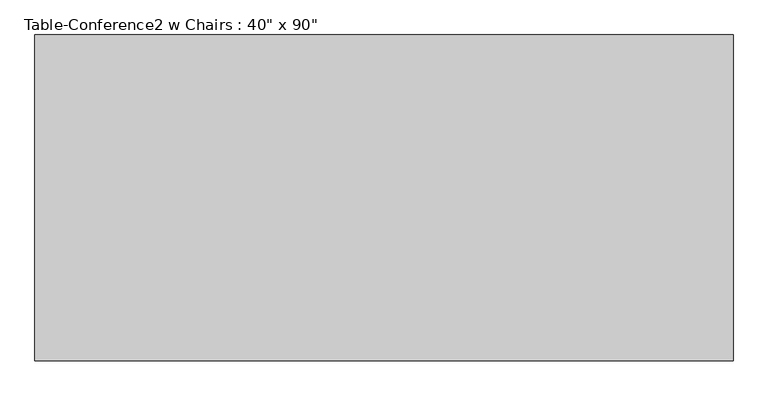
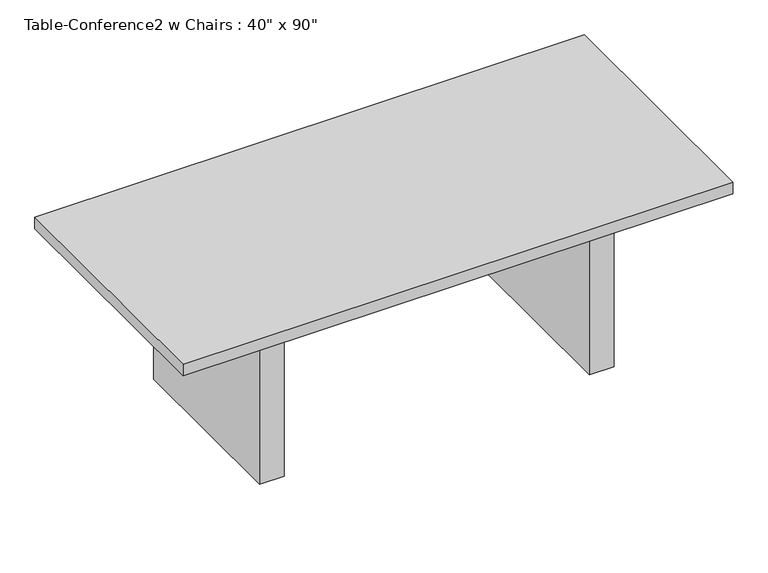
"""IFC4 building model written with IfcOpenShell, lengths in millimetres: furniture geometry."""

import ifcopenshell
import ifcopenshell.guid

model = None  # the IFC model being written
_history = None  # IfcOwnerHistory: only IFC2X3 demands one
_inside = {}  # id of a spatial element -> (the spatial element, [elements in it])
_under = {}  # id of a project, library or spatial element -> (it, [spatial elements below it])
_declared = {}  # id of a project -> (the project, [libraries it declares])
_typed = {}  # id of a type object -> (the type object, [elements of that type])
_made_of = {}  # id of a material, layer set ... -> (it, [elements and type objects made of it])


def new_model(schema):
    """Start an empty IFC model of exactly this schema.

    Asked for "IFC4X3", IfcOpenShell would pick the latest addendum, in which some entities
    have other attributes; the version numbers below select the first issue.
    IFC2X3 requires an IfcOwnerHistory on every rooted entity: one is made here for all.
    """
    global model, _history
    if schema == "IFC4X3":
        model = ifcopenshell.file(schema_version=(4, 3, 0, 0))
    else:
        model = ifcopenshell.file(schema=schema)
    _inside.clear()
    _under.clear()
    _declared.clear()
    _typed.clear()
    _made_of.clear()
    _history = None
    if model.schema == "IFC2X3":
        org = make("IfcOrganization", Name="unknown")
        user = make(
            "IfcPersonAndOrganization",
            ThePerson=make("IfcPerson", FamilyName="unknown"),
            TheOrganization=org,
        )
        app = make(
            "IfcApplication",
            ApplicationDeveloper=org,
            Version="unknown",
            ApplicationFullName="unknown",
            ApplicationIdentifier="unknown",
        )
        _history = make(
            "IfcOwnerHistory",
            OwningUser=user,
            OwningApplication=app,
            ChangeAction="ADDED",
            CreationDate=0,
        )
    return model


def make(cls, **values):
    """One entity of the class cls with the attributes given. An attribute that is None is left unset."""
    return model.create_entity(
        cls, **{name: value for name, value in values.items() if value is not None}
    )


def rooted(cls, **values):
    """An entity with a GlobalId (a new one), such as an element, a storey or a relation."""
    return make(cls, GlobalId=ifcopenshell.guid.new(), OwnerHistory=_history, **values)


def si_unit(unit_type, name, prefix=None):
    """IfcSIUnit, for example si_unit("LENGTHUNIT", "METRE", prefix="MILLI")."""
    return make("IfcSIUnit", UnitType=unit_type, Prefix=prefix, Name=name)


def assignment(units):
    """IfcUnitAssignment: the units of a project."""
    return None if units is None else make("IfcUnitAssignment", Units=units)


def point(xyz):
    """IfcCartesianPoint."""
    return None if xyz is None else make("IfcCartesianPoint", Coordinates=xyz)


def direction(xyz):
    """IfcDirection."""
    return None if xyz is None else make("IfcDirection", DirectionRatios=xyz)


def frame(location, z_axis=None, x_axis=None):
    """IfcAxis2Placement3D, a coordinate frame: its origin and axes. An axis left out is left unset."""
    return make(
        "IfcAxis2Placement3D",
        Location=point(location),
        Axis=direction(z_axis),
        RefDirection=direction(x_axis),
    )


def origin():
    """The frame at (0, 0, 0) with its axes left unset."""
    return frame((0.0, 0.0, 0.0))


def origin_with_axes():
    """The frame at (0, 0, 0) with the z axis (0, 0, 1) and the x axis (1, 0, 0) written out."""
    return frame((0.0, 0.0, 0.0), z_axis=(0.0, 0.0, 1.0), x_axis=(1.0, 0.0, 0.0))


def place(relative_to, where):
    """IfcLocalPlacement: puts the frame where relative to a parent placement (None: the world)."""
    return make(
        "IfcLocalPlacement", PlacementRelTo=relative_to, RelativePlacement=where
    )


def context(
    kind, dimensions, precision=None, world=None, true_north=None, identifier=None
):
    """IfcGeometricRepresentationContext, for example the 3D "Model" context."""
    return make(
        "IfcGeometricRepresentationContext",
        ContextIdentifier=identifier,
        ContextType=kind,
        CoordinateSpaceDimension=dimensions,
        Precision=precision,
        WorldCoordinateSystem=world,
        TrueNorth=true_north,
    )


def project(units=None, contexts=None):
    """IfcProject with its units and contexts."""
    return rooted(
        "IfcProject",
        Name="project",
        RepresentationContexts=contexts,
        UnitsInContext=assignment(units),
    )


def spatial(cls, under=None, at=None, **own):
    """A site, building, storey or space (cls), placed at a placement, below another one or the project."""
    s = rooted(cls, ObjectPlacement=at, **own)
    if under is not None:
        _under.setdefault(under.id(), (under, []))[1].append(s)
    return s


def polyline(points):
    """IfcPolyline through the points."""
    return make("IfcPolyline", Points=[point(p) for p in points])


def outline(outer, holes=None, kind="AREA"):
    """IfcArbitraryClosedProfileDef: a profile drawn as a closed curve; with holes, ...WithVoids."""
    if holes is None:
        return make("IfcArbitraryClosedProfileDef", ProfileType=kind, OuterCurve=outer)
    return make(
        "IfcArbitraryProfileDefWithVoids",
        ProfileType=kind,
        OuterCurve=outer,
        InnerCurves=holes,
    )


def extrude(swept, where, along, depth):
    """IfcExtrudedAreaSolid: the profile swept, set in the frame where, extruded along a direction by depth."""
    return make(
        "IfcExtrudedAreaSolid",
        SweptArea=swept,
        Position=where,
        ExtrudedDirection=direction(along),
        Depth=depth,
    )


def shape(context_of_items, identifier, shape_type, items):
    """IfcShapeRepresentation: the items that make up one representation, for example the "Body"."""
    return make(
        "IfcShapeRepresentation",
        ContextOfItems=context_of_items,
        RepresentationIdentifier=identifier,
        RepresentationType=shape_type,
        Items=items,
    )


def source(mapping_origin, context_of_items, identifier, shape_type, items):
    """IfcRepresentationMap: a shape defined once, which mapped items show again and again."""
    return make(
        "IfcRepresentationMap",
        MappingOrigin=mapping_origin,
        MappedRepresentation=shape(context_of_items, identifier, shape_type, items),
    )


def transform(
    local_origin,
    x_axis=None,
    y_axis=None,
    z_axis=None,
    scale=None,
    scale2=None,
    scale3=None,
    uniform=True,
):
    """IfcCartesianTransformationOperator3D, or its non-uniform kind. x_axis, y_axis, z_axis: its Axis1, 2, 3."""
    if uniform:
        return make(
            "IfcCartesianTransformationOperator3D",
            Axis1=direction(x_axis),
            Axis2=direction(y_axis),
            LocalOrigin=point(local_origin),
            Scale=scale,
            Axis3=direction(z_axis),
        )
    return make(
        "IfcCartesianTransformationOperator3DnonUniform",
        Axis1=direction(x_axis),
        Axis2=direction(y_axis),
        LocalOrigin=point(local_origin),
        Scale=scale,
        Axis3=direction(z_axis),
        Scale2=scale2,
        Scale3=scale3,
    )


def mapped(mapping_source, mapping_target):
    """IfcMappedItem: shows the shape of a source again, moved by a transform."""
    return make(
        "IfcMappedItem", MappingSource=mapping_source, MappingTarget=mapping_target
    )


def made_of(thing, what):
    """Note that an element or type object is made of a material, layer set ...; save() writes the relation."""
    if what is not None:
        _made_of.setdefault(what.id(), (what, []))[1].append(thing)
    return thing


def element(
    cls,
    number,
    at=None,
    inside=None,
    cuts=None,
    type_object=None,
    material=None,
    context=None,
    identifier="Body",
    shape_type=None,
    held_by="IfcProductDefinitionShape",
    body=None,
    shapes=None,
    **own,
):
    """One element of the class cls, such as IfcWall. Its Tag is "e" and its number.

    at: its placement. inside: the storey or other place that contains it. cuts: it is an
    opening in that element (IfcRelVoidsElement). A single representation is given by context,
    identifier, shape_type and body (its items); several are given by shapes. held_by: the class
    of the entity that holds the representations. save() writes the other relations.
    """
    e = rooted(cls, Tag="e%d" % number, ObjectPlacement=at, **own)
    if body is not None:
        shapes = [shape(context, identifier, shape_type, body)]
    if shapes is not None:
        e.Representation = make(held_by, Representations=shapes)
    if inside is not None:
        _inside.setdefault(inside.id(), (inside, []))[1].append(e)
    if cuts is not None:
        rooted(
            "IfcRelVoidsElement", RelatingBuildingElement=cuts, RelatedOpeningElement=e
        )
    if type_object is not None:
        _typed.setdefault(type_object.id(), (type_object, []))[1].append(e)
    return made_of(e, material)


def aggregate(whole, parts):
    """IfcRelAggregates: a whole, such as a stair, and the parts it consists of."""
    return rooted("IfcRelAggregates", RelatingObject=whole, RelatedObjects=parts)


def save(model, path):
    """Write the relations noted so far, then the file.

    IfcRelAggregates (storeys below a building ...), IfcRelContainedInSpatialStructure (elements
    in a storey), IfcRelDefinesByType, IfcRelAssociatesMaterial and IfcRelDeclares: one each for
    every whole, place, type object, material and project.
    """
    for whole, parts in _under.values():
        aggregate(whole, parts)
    for where, things in _inside.values():
        rooted(
            "IfcRelContainedInSpatialStructure",
            RelatedElements=things,
            RelatingStructure=where,
        )
    for kind, things in _typed.values():
        rooted("IfcRelDefinesByType", RelatedObjects=things, RelatingType=kind)
    for what, things in _made_of.values():
        rooted("IfcRelAssociatesMaterial", RelatedObjects=things, RelatingMaterial=what)
    for by, libraries in _declared.values():
        rooted("IfcRelDeclares", RelatingContext=by, RelatedDefinitions=libraries)
    model.write(path)


def furniture_ed4cefae(model_context):
    return source(origin(), model_context, "Body", "SweptSolid", [
        extrude(outline(polyline([(635.0, 381.0), (635.0, 342.9), (-635.0, 342.9), (-635.0, 381.0), (635.0, 381.0)])), frame((0.0, 0.0, 609.6), z_axis=(0.0, 0.0, 1.0), x_axis=(1.0, 0.0, 0.0)), (0.0, 0.0, 1.0), 101.6),
        extrude(outline(polyline([(635.0, -381.0), (-635.0, -381.0), (-635.0, -342.9), (635.0, -342.9), (635.0, -381.0)])), frame((0.0, 0.0, 609.6), z_axis=(0.0, 0.0, 1.0), x_axis=(1.0, 0.0, 0.0)), (0.0, 0.0, 1.0), 101.6),
        extrude(outline(polyline([(-635.0, -381.0), (-736.6, -381.0), (-736.6, 381.0), (-635.0, 381.0), (-635.0, -381.0)])), origin_with_axes(), (0.0, 0.0, 1.0), 711.2),
        extrude(outline(polyline([(736.6, -381.0), (635.0, -381.0), (635.0, 381.0), (736.6, 381.0), (736.6, -381.0)])), origin_with_axes(), (0.0, 0.0, 1.0), 711.2),
        extrude(outline(polyline([(1143.0, -533.4), (-1143.0, -533.4), (-1143.0, 533.4), (1143.0, 533.4), (1143.0, -533.4)])), frame((0.0, 0.0, 711.2), z_axis=(0.0, 0.0, 1.0), x_axis=(1.0, 0.0, 0.0)), (0.0, 0.0, 1.0), 50.8),
    ])


if __name__ == "__main__":
    model = new_model("IFC4")
    model_context = context("Model", 3, world=origin())
    ifc_project = project(units=[si_unit("LENGTHUNIT", "METRE", prefix="MILLI")], contexts=[model_context])
    site = spatial("IfcSite", under=ifc_project)
    building = spatial("IfcBuilding", under=site)
    placement = place(None, origin())
    furniture_shape = furniture_ed4cefae(model_context)
    element("IfcFurniture", 1, ObjectType="Table-Conference2 w Chairs : 40\" x 90\"", at=placement, inside=building, context=model_context, shape_type="MappedRepresentation", body=[
        mapped(furniture_shape, transform((0.0, 0.0, 0.0), x_axis=(1.0, 0.0, 0.0), y_axis=(0.0, 1.0, 0.0), z_axis=(0.0, 0.0, 1.0))),
    ])
    save(model, "model.ifc")

# Revit data of these elements
# Type "Table-Conference2 w Chairs : 40\" x 90\""
#   Type IfcGUID = "2u0XNFrAPALBFZCv81fqic"
#   Assembly Code = "E2020200"
#   Description = "Seating 6-8"
#   Height = 0.762 m
#   Length = 2.286 m
#   Width = 1.0668 m
#   Number Of Chairs One Side = 3
#   Number Of Chairs = 8
#   Material = Wood - Cherry
#   Default Elevation = 0
# Element 1 (IfcFurniture, "Table-Conference2 w Chairs : 40\" x 90\"")
#   Materials on its faces: "Wood - Cherry"
# Materials
#   "Wood - Cherry": class "Wood", colour RGB 226 177 128, transparency 0
